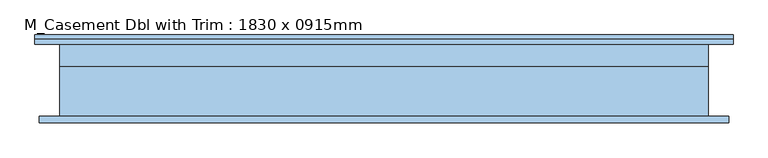
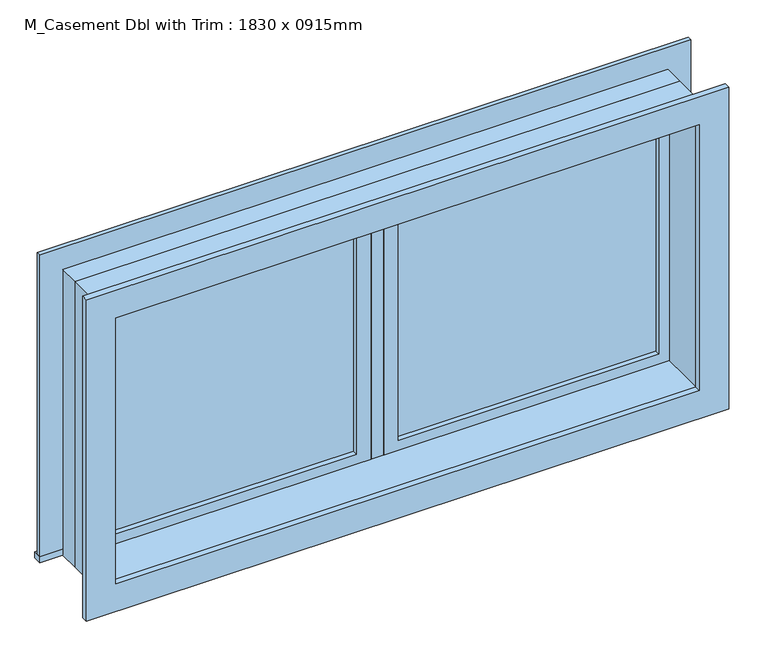
"""IFC4 building model written with IfcOpenShell, lengths in millimetres: window geometry, M_Casement Dbl with Trim : 1830 x 0915mm."""

import ifcopenshell
import ifcopenshell.guid

model = None  # the IFC model being written
_history = None  # IfcOwnerHistory: only IFC2X3 demands one
_inside = {}  # id of a spatial element -> (the spatial element, [elements in it])
_under = {}  # id of a project, library or spatial element -> (it, [spatial elements below it])
_declared = {}  # id of a project -> (the project, [libraries it declares])
_typed = {}  # id of a type object -> (the type object, [elements of that type])
_made_of = {}  # id of a material, layer set ... -> (it, [elements and type objects made of it])


def new_model(schema):
    """Start an empty IFC model of exactly this schema.

    Asked for "IFC4X3", IfcOpenShell would pick the latest addendum, in which some entities
    have other attributes; the version numbers below select the first issue.
    IFC2X3 requires an IfcOwnerHistory on every rooted entity: one is made here for all.
    """
    global model, _history
    if schema == "IFC4X3":
        model = ifcopenshell.file(schema_version=(4, 3, 0, 0))
    else:
        model = ifcopenshell.file(schema=schema)
    _inside.clear()
    _under.clear()
    _declared.clear()
    _typed.clear()
    _made_of.clear()
    _history = None
    if model.schema == "IFC2X3":
        org = make("IfcOrganization", Name="unknown")
        user = make(
            "IfcPersonAndOrganization",
            ThePerson=make("IfcPerson", FamilyName="unknown"),
            TheOrganization=org,
        )
        app = make(
            "IfcApplication",
            ApplicationDeveloper=org,
            Version="unknown",
            ApplicationFullName="unknown",
            ApplicationIdentifier="unknown",
        )
        _history = make(
            "IfcOwnerHistory",
            OwningUser=user,
            OwningApplication=app,
            ChangeAction="ADDED",
            CreationDate=0,
        )
    return model


def make(cls, **values):
    """One entity of the class cls with the attributes given. An attribute that is None is left unset."""
    return model.create_entity(
        cls, **{name: value for name, value in values.items() if value is not None}
    )


def rooted(cls, **values):
    """An entity with a GlobalId (a new one), such as an element, a storey or a relation."""
    return make(cls, GlobalId=ifcopenshell.guid.new(), OwnerHistory=_history, **values)


def si_unit(unit_type, name, prefix=None):
    """IfcSIUnit, for example si_unit("LENGTHUNIT", "METRE", prefix="MILLI")."""
    return make("IfcSIUnit", UnitType=unit_type, Prefix=prefix, Name=name)


def assignment(units):
    """IfcUnitAssignment: the units of a project."""
    return None if units is None else make("IfcUnitAssignment", Units=units)


def point(xyz):
    """IfcCartesianPoint."""
    return None if xyz is None else make("IfcCartesianPoint", Coordinates=xyz)


def direction(xyz):
    """IfcDirection."""
    return None if xyz is None else make("IfcDirection", DirectionRatios=xyz)


def frame(location, z_axis=None, x_axis=None):
    """IfcAxis2Placement3D, a coordinate frame: its origin and axes. An axis left out is left unset."""
    return make(
        "IfcAxis2Placement3D",
        Location=point(location),
        Axis=direction(z_axis),
        RefDirection=direction(x_axis),
    )


def origin():
    """The frame at (0, 0, 0) with its axes left unset."""
    return frame((0.0, 0.0, 0.0))


def place(relative_to, where):
    """IfcLocalPlacement: puts the frame where relative to a parent placement (None: the world)."""
    return make(
        "IfcLocalPlacement", PlacementRelTo=relative_to, RelativePlacement=where
    )


def context(
    kind, dimensions, precision=None, world=None, true_north=None, identifier=None
):
    """IfcGeometricRepresentationContext, for example the 3D "Model" context."""
    return make(
        "IfcGeometricRepresentationContext",
        ContextIdentifier=identifier,
        ContextType=kind,
        CoordinateSpaceDimension=dimensions,
        Precision=precision,
        WorldCoordinateSystem=world,
        TrueNorth=true_north,
    )


def project(units=None, contexts=None):
    """IfcProject with its units and contexts."""
    return rooted(
        "IfcProject",
        Name="project",
        RepresentationContexts=contexts,
        UnitsInContext=assignment(units),
    )


def spatial(cls, under=None, at=None, **own):
    """A site, building, storey or space (cls), placed at a placement, below another one or the project."""
    s = rooted(cls, ObjectPlacement=at, **own)
    if under is not None:
        _under.setdefault(under.id(), (under, []))[1].append(s)
    return s


def polyline(points):
    """IfcPolyline through the points."""
    return make("IfcPolyline", Points=[point(p) for p in points])


def outline(outer, holes=None, kind="AREA"):
    """IfcArbitraryClosedProfileDef: a profile drawn as a closed curve; with holes, ...WithVoids."""
    if holes is None:
        return make("IfcArbitraryClosedProfileDef", ProfileType=kind, OuterCurve=outer)
    return make(
        "IfcArbitraryProfileDefWithVoids",
        ProfileType=kind,
        OuterCurve=outer,
        InnerCurves=holes,
    )


def extrude(swept, where, along, depth):
    """IfcExtrudedAreaSolid: the profile swept, set in the frame where, extruded along a direction by depth."""
    return make(
        "IfcExtrudedAreaSolid",
        SweptArea=swept,
        Position=where,
        ExtrudedDirection=direction(along),
        Depth=depth,
    )


def shape(context_of_items, identifier, shape_type, items):
    """IfcShapeRepresentation: the items that make up one representation, for example the "Body"."""
    return make(
        "IfcShapeRepresentation",
        ContextOfItems=context_of_items,
        RepresentationIdentifier=identifier,
        RepresentationType=shape_type,
        Items=items,
    )


def source(mapping_origin, context_of_items, identifier, shape_type, items):
    """IfcRepresentationMap: a shape defined once, which mapped items show again and again."""
    return make(
        "IfcRepresentationMap",
        MappingOrigin=mapping_origin,
        MappedRepresentation=shape(context_of_items, identifier, shape_type, items),
    )


def transform(
    local_origin,
    x_axis=None,
    y_axis=None,
    z_axis=None,
    scale=None,
    scale2=None,
    scale3=None,
    uniform=True,
):
    """IfcCartesianTransformationOperator3D, or its non-uniform kind. x_axis, y_axis, z_axis: its Axis1, 2, 3."""
    if uniform:
        return make(
            "IfcCartesianTransformationOperator3D",
            Axis1=direction(x_axis),
            Axis2=direction(y_axis),
            LocalOrigin=point(local_origin),
            Scale=scale,
            Axis3=direction(z_axis),
        )
    return make(
        "IfcCartesianTransformationOperator3DnonUniform",
        Axis1=direction(x_axis),
        Axis2=direction(y_axis),
        LocalOrigin=point(local_origin),
        Scale=scale,
        Axis3=direction(z_axis),
        Scale2=scale2,
        Scale3=scale3,
    )


def mapped(mapping_source, mapping_target):
    """IfcMappedItem: shows the shape of a source again, moved by a transform."""
    return make(
        "IfcMappedItem", MappingSource=mapping_source, MappingTarget=mapping_target
    )


def made_of(thing, what):
    """Note that an element or type object is made of a material, layer set ...; save() writes the relation."""
    if what is not None:
        _made_of.setdefault(what.id(), (what, []))[1].append(thing)
    return thing


def element(
    cls,
    number,
    at=None,
    inside=None,
    cuts=None,
    type_object=None,
    material=None,
    context=None,
    identifier="Body",
    shape_type=None,
    held_by="IfcProductDefinitionShape",
    body=None,
    shapes=None,
    **own,
):
    """One element of the class cls, such as IfcWall. Its Tag is "e" and its number.

    at: its placement. inside: the storey or other place that contains it. cuts: it is an
    opening in that element (IfcRelVoidsElement). A single representation is given by context,
    identifier, shape_type and body (its items); several are given by shapes. held_by: the class
    of the entity that holds the representations. save() writes the other relations.
    """
    e = rooted(cls, Tag="e%d" % number, ObjectPlacement=at, **own)
    if body is not None:
        shapes = [shape(context, identifier, shape_type, body)]
    if shapes is not None:
        e.Representation = make(held_by, Representations=shapes)
    if inside is not None:
        _inside.setdefault(inside.id(), (inside, []))[1].append(e)
    if cuts is not None:
        rooted(
            "IfcRelVoidsElement", RelatingBuildingElement=cuts, RelatedOpeningElement=e
        )
    if type_object is not None:
        _typed.setdefault(type_object.id(), (type_object, []))[1].append(e)
    return made_of(e, material)


def aggregate(whole, parts):
    """IfcRelAggregates: a whole, such as a stair, and the parts it consists of."""
    return rooted("IfcRelAggregates", RelatingObject=whole, RelatedObjects=parts)


def save(model, path):
    """Write the relations noted so far, then the file.

    IfcRelAggregates (storeys below a building ...), IfcRelContainedInSpatialStructure (elements
    in a storey), IfcRelDefinesByType, IfcRelAssociatesMaterial and IfcRelDeclares: one each for
    every whole, place, type object, material and project.
    """
    for whole, parts in _under.values():
        aggregate(whole, parts)
    for where, things in _inside.values():
        rooted(
            "IfcRelContainedInSpatialStructure",
            RelatedElements=things,
            RelatingStructure=where,
        )
    for kind, things in _typed.values():
        rooted("IfcRelDefinesByType", RelatedObjects=things, RelatingType=kind)
    for what, things in _made_of.values():
        rooted("IfcRelAssociatesMaterial", RelatedObjects=things, RelatingMaterial=what)
    for by, libraries in _declared.values():
        rooted("IfcRelDeclares", RelatingContext=by, RelatedDefinitions=libraries)
    model.write(path)


def m_casement_dbl_with_trim_1830_x_0915mm_5bb5ad82(model_context):
    return source(origin(), model_context, "Body", "SweptSolid", [
        extrude(outline(polyline([(63.5, 85.775), (851.5, 85.775), (851.5, 73.075), (63.5, 73.075), (63.5, 85.775)])), frame((0.0, 0.0, 1283.5), z_axis=(0.0, 0.0, 1.0), x_axis=(1.0, 0.0, 0.0)), (0.0, 0.0, 1.0), 788.0),
        extrude(outline(polyline([(2115.95, 19.05), (1239.05, 19.05), (1239.05, 895.95), (2115.95, 895.95), (2115.95, 19.05)]), holes=[polyline([(2071.5, 63.5), (2071.5, 851.5), (1283.5, 851.5), (1283.5, 63.5), (2071.5, 63.5)])]), frame((0.0, 57.2, 0.0), z_axis=(0.0, 1.0, 0.0), x_axis=(0.0, 0.0, 1.0)), (0.0, 0.0, 1.0), 44.45),
        extrude(outline(polyline([(-984.95, 146.35), (984.95, 146.35), (984.95, 120.65), (-984.95, 120.65), (-984.95, 146.35)])), frame((0.0, 0.0, 1220.0), z_axis=(0.0, 0.0, 1.0), x_axis=(1.0, 0.0, 0.0)), (0.0, 0.0, 1.0), 19.05),
        extrude(outline(polyline([(2115.95, -895.95), (2115.95, 895.95), (1239.05, 895.95), (1239.05, 984.95), (2204.95, 984.95), (2204.95, -984.95), (1239.05, -984.95), (1239.05, -895.95), (2115.95, -895.95)])), frame((0.0, 120.65, 0.0), z_axis=(0.0, 1.0, 0.0), x_axis=(0.0, 0.0, 1.0)), (0.0, 0.0, 1.0), 13.0),
        extrude(outline(polyline([(2192.25, 972.25), (2192.25, -972.25), (1162.75, -972.25), (1162.75, 972.25), (2192.25, 972.25)]), holes=[polyline([(2103.25, 883.25), (1251.75, 883.25), (1251.75, -883.25), (2103.25, -883.25), (2103.25, 883.25)])]), frame((0.0, -101.55, 0.0), z_axis=(0.0, 1.0, 0.0), x_axis=(0.0, 0.0, 1.0)), (0.0, 0.0, 1.0), 19.0),
        extrude(outline(polyline([(-63.5, 73.075), (-851.5, 73.075), (-851.5, 85.775), (-63.5, 85.775), (-63.5, 73.075)])), frame((0.0, 0.0, 1283.5), z_axis=(0.0, 0.0, 1.0), x_axis=(1.0, 0.0, 0.0)), (0.0, 0.0, 1.0), 788.0),
        extrude(outline(polyline([(2115.95, -895.95), (1239.05, -895.95), (1239.05, -19.05), (2115.95, -19.05), (2115.95, -895.95)]), holes=[polyline([(2071.5, -851.5), (2071.5, -63.5), (1283.5, -63.5), (1283.5, -851.5), (2071.5, -851.5)])]), frame((0.0, 57.2, 0.0), z_axis=(0.0, 1.0, 0.0), x_axis=(0.0, 0.0, 1.0)), (0.0, 0.0, 1.0), 44.45),
        extrude(outline(polyline([(2135.0, -915.0), (1220.0, -915.0), (1220.0, 915.0), (2135.0, 915.0), (2135.0, -915.0)]), holes=[polyline([(2103.25, -883.25), (2103.25, 883.25), (1251.75, 883.25), (1251.75, -883.25), (2103.25, -883.25)])]), frame((0.0, -82.55, 0.0), z_axis=(0.0, 1.0, 0.0), x_axis=(0.0, 0.0, 1.0)), (0.0, 0.0, 1.0), 139.75),
        extrude(outline(polyline([(2135.0, 915.0), (2135.0, -915.0), (1220.0, -915.0), (1220.0, 915.0), (2135.0, 915.0)]), holes=[polyline([(2115.95, 895.95), (1239.05, 895.95), (1239.05, -895.95), (2115.95, -895.95), (2115.95, 895.95)])]), frame((0.0, 57.2, 0.0), z_axis=(0.0, 1.0, 0.0), x_axis=(0.0, 0.0, 1.0)), (0.0, 0.0, 1.0), 63.45),
        extrude(outline(polyline([(19.05, 57.2), (-19.05, 57.2), (-19.05, 120.7), (19.05, 120.7), (19.05, 57.2)])), frame((0.0, 0.0, 1239.05), z_axis=(0.0, 0.0, 1.0), x_axis=(1.0, 0.0, 0.0)), (0.0, 0.0, 1.0), 876.9),
    ])


if __name__ == "__main__":
    model = new_model("IFC4")
    model_context = context("Model", 3, world=origin())
    ifc_project = project(units=[si_unit("LENGTHUNIT", "METRE", prefix="MILLI")], contexts=[model_context])
    site = spatial("IfcSite", under=ifc_project)
    building = spatial("IfcBuilding", under=site)
    placement = place(None, origin())
    m_casement_dbl_with_trim_1830_x_0915mm_shape = m_casement_dbl_with_trim_1830_x_0915mm_5bb5ad82(model_context)
    element("IfcWindow", 1, ObjectType="M_Casement Dbl with Trim : 1830 x 0915mm", at=placement, inside=building, context=model_context, shape_type="MappedRepresentation", body=[
        mapped(m_casement_dbl_with_trim_1830_x_0915mm_shape, transform((0.0, 0.0, 0.0), x_axis=(1.0, 0.0, 0.0), y_axis=(0.0, 1.0, 0.0), z_axis=(0.0, 0.0, 1.0))),
    ])
    save(model, "model.ifc")

# Revit data of these elements
# Type "M_Casement Dbl with Trim : 1830 x 0915mm"
#   Type Mark = "23"
#   Construction Type Id = "GSP4R"
#   Analytic Construction = "1/8 in Pilkington single glazing"
#   Visual Light Transmittance = 0.9
#   Solar Heat Gain Coefficient = 0.78
#   Heat Transfer Coefficient (U) = 3.6886 W/(m²·K)
#   Height = 915 mm
#   Default Sill Height = 1220 mm
#   Trim Projection - Ext. = 13 mm
#   Trim Projection - Int. = 19 mm
#   Trim Width - Exterior = 89 mm
#   Trim Width - Interior = 89 mm
#   Width = 1830 mm
#   Window Inset = 19 mm
#   Glass Pane Material = Glass
#   Sash = Sash
#   Trim Exterior Material = Trim
#   Trim Interior Material = Trim
#   Wall Closure = (empty or 0)
# Element 1 (IfcWindow, "M_Casement Dbl with Trim : 1830 x 0915mm")
#   Materials on its faces: "Trim", "Sash", "Glass"
# Materials
#   "Glass": class "Glass", colour RGB 0 128 192, transparency 0.75, Description = "Soda Lime Glass", Cost = 0
#   "Sash": class "Wood", colour RGB 224 178 126, transparency 0, Cost = 0
#   "Trim": class "Wood", colour RGB 224 178 126, transparency 0
